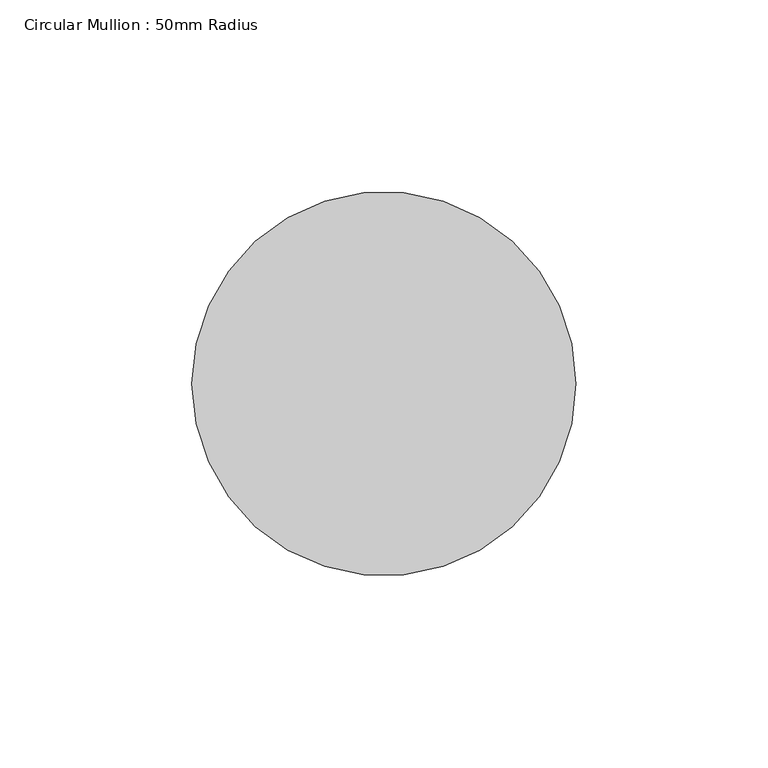
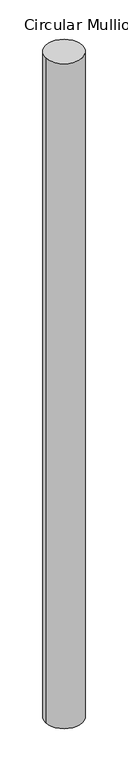
"""IFC4 building model written with IfcOpenShell, lengths in millimetres: member geometry, Circular Mullion : 50mm Radius."""

from ifc_helpers import new_model, si_unit, point, frame, frame_2d, origin, place, context, project, spatial, circle_curve, trimmed, segment, composite_curve, outline, extrude, source, transform, mapped, element, save


def circular_mullion_50mm_radius_94a3c504(model_context):
    return source(origin(), model_context, "Body", "SweptSolid", [
        extrude(outline(composite_curve([segment(trimmed(circle_curve(frame_2d((-50.0, 0.0)), 50.0), [point((0.0, 0.0))], [point((-100.0, 0.0))], False, "CARTESIAN"), True, "CONTINUOUS"), segment(trimmed(circle_curve(frame_2d((-50.0, 0.0)), 50.0), [point((-100.0, 0.0))], [point((0.0, 0.0))], False, "CARTESIAN"), True, "CONTINUOUS")], self_intersect=False)), frame((0.0, 0.0, -1904.8171937), z_axis=(0.0, 0.0, 1.0), x_axis=(1.0, 0.0, 0.0)), (0.0, 0.0, 1.0), 1904.8171937),
    ])


if __name__ == "__main__":
    model = new_model("IFC4")
    model_context = context("Model", 3, world=origin())
    ifc_project = project(units=[si_unit("LENGTHUNIT", "METRE", prefix="MILLI")], contexts=[model_context])
    site = spatial("IfcSite", under=ifc_project)
    building = spatial("IfcBuilding", under=site)
    placement = place(None, origin())
    circular_mullion_50mm_radius_shape = circular_mullion_50mm_radius_94a3c504(model_context)
    element("IfcMember", 1, ObjectType="Circular Mullion : 50mm Radius", at=placement, inside=building, context=model_context, shape_type="MappedRepresentation", body=[
        mapped(circular_mullion_50mm_radius_shape, transform((0.0, 0.0, 0.0), x_axis=(1.0, 0.0, 0.0), y_axis=(0.0, 1.0, 0.0), z_axis=(0.0, 0.0, 1.0))),
    ])
    save(model, "model.ifc")

# Revit data of these elements
# Type "Circular Mullion : 50mm Radius"
#   built-in parameter 1007350 = 0.164042 (stored number, unit not read)
# Element 1 (IfcMember, "Circular Mullion : 50mm Radius")
#   Materials on its faces: "Aluminium"
# Materials
#   "Aluminium": class "Metal", colour RGB 247 247 247, transparency 0, Description = "Aluminium 6061", Cost = 0
